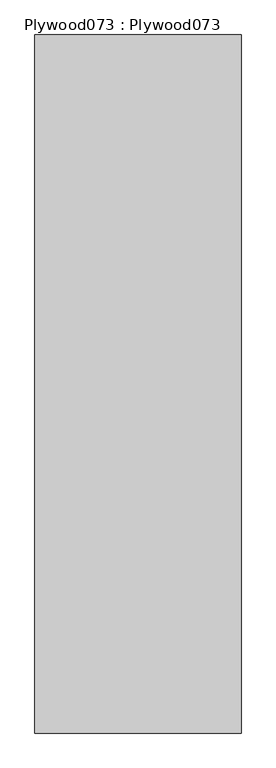
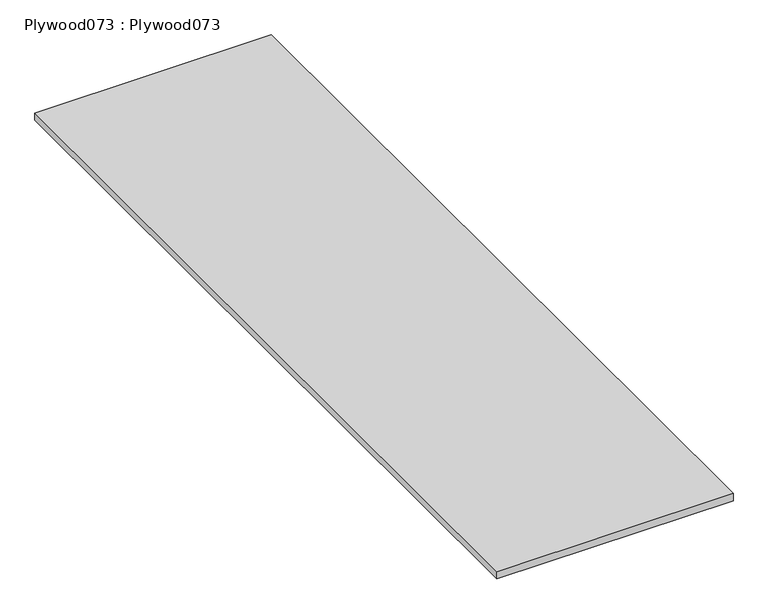
"""IFC4 building model written with IfcOpenShell, lengths in millimetres: proxy geometry, Plywood073 : Plywood073."""

from ifc_helpers import new_model, si_unit, frame, origin, place, context, project, spatial, polyline, outline, extrude, source, transform, mapped, element, save


def plywood073_plywood073_11937f15(model_context):
    return source(origin(), model_context, "Body", "SweptSolid", [
        extrude(outline(polyline([(-4404.2038825, -1052.8906574), (-4994.7538825, -1052.8906574), (-4994.7538825, 947.1093426), (-4404.2038825, 947.1093426), (-4404.2038825, -1052.8906574)])), frame((0.0, 0.0, 39560.2460083), z_axis=(0.0, 0.0, 1.0), x_axis=(1.0, 0.0, 0.0)), (0.0, 0.0, 1.0), 19.05),
    ])


if __name__ == "__main__":
    model = new_model("IFC4")
    model_context = context("Model", 3, world=origin())
    ifc_project = project(units=[si_unit("LENGTHUNIT", "METRE", prefix="MILLI")], contexts=[model_context])
    site = spatial("IfcSite", under=ifc_project)
    building = spatial("IfcBuilding", under=site)
    placement = place(None, origin())
    plywood073_plywood073_shape = plywood073_plywood073_11937f15(model_context)
    element("IfcBuildingElementProxy", 1, Name="Plywood073 : Plywood073", ObjectType="Plywood073 : Plywood073", at=placement, inside=building, context=model_context, shape_type="MappedRepresentation", body=[
        mapped(plywood073_plywood073_shape, transform((0.0, 0.0, 0.0), x_axis=(1.0, 0.0, 0.0), y_axis=(0.0, 1.0, 0.0), z_axis=(0.0, 0.0, 1.0))),
    ])
    save(model, "model.ifc")

# Revit data of these elements
# Type "Plywood073 : Plywood073"
#   NameOverride = "Plywood073"
# Element 1 (IfcBuildingElementProxy, "Plywood073 : Plywood073")
#   Materials on its faces: "CDX PLYWOOD -  SEE STRUCTURAL DWGS"
# Materials
#   "CDX PLYWOOD -  SEE STRUCTURAL DWGS": class "Unassigned", colour RGB 177 130 114, transparency 0, Cost = 0
